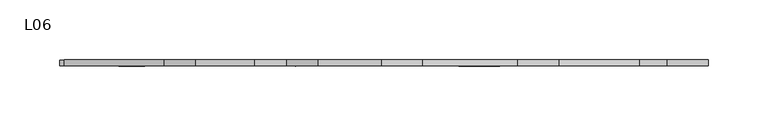
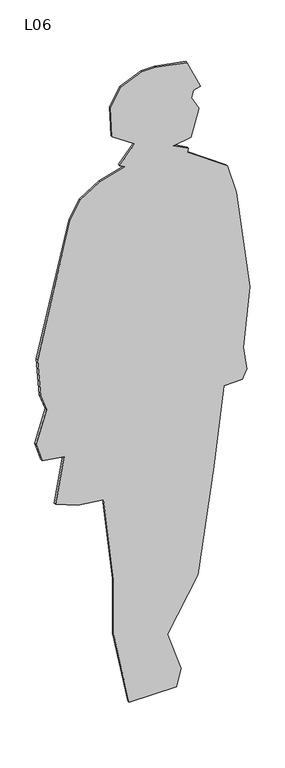
"""IFC4 building model written with IfcOpenShell, lengths in millimetres: proxy geometry, 09_Lady_06 : L06."""

from ifc_helpers import new_model, si_unit, frame, origin, place, context, project, spatial, polyline, outline, extrude, source, transform, mapped, element, save


def l06_b6015df7(model_context):
    return source(origin(), model_context, "Body", "SweptSolid", [
        extrude(outline(polyline([(996.4350196, -292.882987), (897.9071039, -285.3039227), (856.2220924, -270.145794), (772.8523845, -296.6724408), (723.5883087, -281.5143121), (714.3060978, -225.8209501), (594.7438996, -247.4086009), (572.0067852, -190.5654607), (564.030361, -125.3176962), (340.8450071, -99.6163739), (194.8893637, -100.0244772), (0.0, -60.2928032), (0.0, 59.1056173), (45.2608677, 70.9128107), (147.578394, 36.8070209), (280.1990069, 113.1642476), (555.2775152, 154.4259527), (762.8264301, 178.9713291), (762.8264301, 226.3723793), (777.3024197, 232.1628535), (785.9881704, 237.9532491), (848.6428707, 228.5575067), (1004.0140048, 245.2316059), (1269.28173, 211.1256588), (1348.0395708, 187.9615595), (1418.7743591, 87.4435479), (1428.4420033, 89.8604713), (1449.3332407, 52.256712), (1456.6743202, 96.3027321), (1526.9701544, 116.3871968), (1561.075787, 97.4395357), (1580.1193607, 102.9388568), (1583.813216, 120.1767293), (1659.6039387, 86.0709394), (1674.7622247, 6.4906848), (1674.7622247, -27.6151837), (1652.0250316, -80.6687914), (1606.550409, -107.1954383), (1526.9701544, -103.4059845), (1489.0749113, -46.5629229), (1443.6002893, -84.4582452), (1435.5225039, -70.9955118), (1417.0735638, -133.7223205), (1386.7572277, -182.9863964), (1341.2828416, -209.5129646), (996.4350196, -292.882987)])), frame((0.0, -5.0, 0.0), z_axis=(0.0, 1.0, 0.0), x_axis=(0.0, 0.0, 1.0)), (0.0, 0.0, 1.0), 5.0),
    ])


if __name__ == "__main__":
    model = new_model("IFC4")
    model_context = context("Model", 3, world=origin())
    ifc_project = project(units=[si_unit("LENGTHUNIT", "METRE", prefix="MILLI")], contexts=[model_context])
    site = spatial("IfcSite", under=ifc_project)
    building = spatial("IfcBuilding", under=site)
    placement = place(None, origin())
    l06_shape = l06_b6015df7(model_context)
    element("IfcBuildingElementProxy", 1, Name="09_Lady_06 : L06", ObjectType="09_Lady_06 : L06", at=placement, inside=building, context=model_context, shape_type="MappedRepresentation", body=[
        mapped(l06_shape, transform((0.0, 0.0, 0.0), x_axis=(1.0, 0.0, 0.0), y_axis=(0.0, 1.0, 0.0), z_axis=(0.0, 0.0, 1.0))),
    ])
    save(model, "model.ifc")

# Revit data of these elements
# Type "09_Lady_06 : L06"
#   Flat Material = none
#   Height = 0
